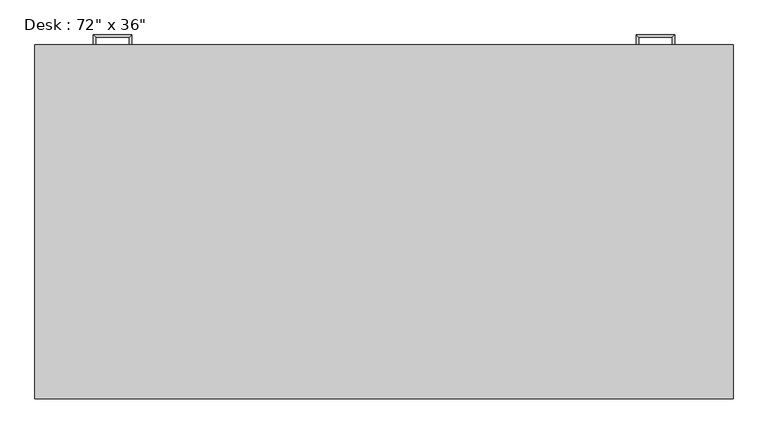
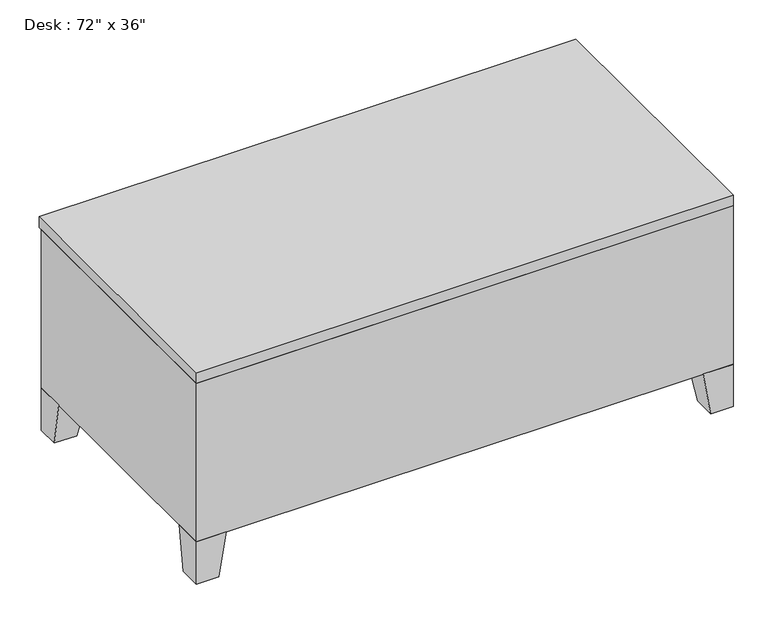
"""IFC4 building model written with IfcOpenShell, lengths in millimetres: furniture geometry."""

from ifc_helpers import new_model, si_unit, frame, origin, place, context, project, spatial, polyline, outline, extrude, faceted_brep, source, transform, mapped, element, save


def furniture_65204735(model_context):
    return source(origin(), model_context, "Body", "SolidModel", [
        extrude(outline(polyline([(-133.35, 76.2), (-133.35, 88.9), (234.95, 88.9), (234.95, 76.2), (-133.35, 76.2)])), frame((0.0, 0.0, 603.25), z_axis=(0.0, 0.0, 1.0), x_axis=(1.0, 0.0, 0.0)), (0.0, 0.0, 1.0), 101.6),
        extrude(outline(polyline([(-133.35, 76.2), (-133.35, 88.9), (234.95, 88.9), (234.95, 76.2), (-133.35, 76.2)])), frame((0.0, 0.0, 171.45), z_axis=(0.0, 0.0, 1.0), x_axis=(1.0, 0.0, 0.0)), (0.0, 0.0, 1.0), 412.75),
        extrude(outline(polyline([(1289.05, 76.2), (1289.05, 88.9), (1657.35, 88.9), (1657.35, 76.2), (1289.05, 76.2)])), frame((0.0, 0.0, 603.25), z_axis=(0.0, 0.0, 1.0), x_axis=(1.0, 0.0, 0.0)), (0.0, 0.0, 1.0), 101.6),
        extrude(outline(polyline([(1289.05, 76.2), (1289.05, 88.9), (1657.35, 88.9), (1657.35, 76.2), (1289.05, 76.2)])), frame((0.0, 0.0, 171.45), z_axis=(0.0, 0.0, 1.0), x_axis=(1.0, 0.0, 0.0)), (0.0, 0.0, 1.0), 171.45),
        extrude(outline(polyline([(1289.05, 76.2), (1289.05, 88.9), (1657.35, 88.9), (1657.35, 76.2), (1289.05, 76.2)])), frame((0.0, 0.0, 482.6), z_axis=(0.0, 0.0, 1.0), x_axis=(1.0, 0.0, 0.0)), (0.0, 0.0, 1.0), 101.6),
        extrude(outline(polyline([(1289.05, 76.2), (1289.05, 88.9), (1657.35, 88.9), (1657.35, 76.2), (1289.05, 76.2)])), frame((0.0, 0.0, 361.95), z_axis=(0.0, 0.0, 1.0), x_axis=(1.0, 0.0, 0.0)), (0.0, 0.0, 1.0), 101.6),
        faceted_brep([(-50.8, 76.2, 152.4), (-152.4, 76.2, 152.4), (-152.4, -25.4, 152.4), (-50.8, -25.4, 152.4), (-76.2, 76.2, 0.0), (-76.2, 0.0, 0.0), (-152.4, 0.0, 0.0), (-152.4, 76.2, 0.0)], [[[0, 1, 2, 3]], [[4, 5, 6, 7]], [[4, 0, 3, 5]], [[5, 3, 2, 6]], [[6, 2, 1, 7]], [[7, 1, 0, 4]]]),
        faceted_brep([(-50.8, -838.2, 152.4), (-50.8, -736.6, 152.4), (-152.4, -736.6, 152.4), (-152.4, -838.2, 152.4), (-76.2, -838.2, 0.0), (-152.4, -838.2, 0.0), (-152.4, -762.0, 0.0), (-76.2, -762.0, 0.0)], [[[0, 1, 2, 3]], [[4, 5, 6, 7]], [[4, 0, 3, 5]], [[5, 3, 2, 6]], [[6, 2, 1, 7]], [[7, 1, 0, 4]]]),
        faceted_brep([(1574.8, -838.2, 152.4), (1676.4, -838.2, 152.4), (1676.4, -736.6, 152.4), (1574.8, -736.6, 152.4), (1600.2, -838.2, 0.0), (1600.2, -762.0, 0.0), (1676.4, -762.0, 0.0), (1676.4, -838.2, 0.0)], [[[0, 1, 2, 3]], [[4, 5, 6, 7]], [[4, 0, 3, 5]], [[5, 3, 2, 6]], [[6, 2, 1, 7]], [[7, 1, 0, 4]]]),
        faceted_brep([(1574.8, 76.2, 152.4), (1574.8, -25.4, 152.4), (1676.4, -25.4, 152.4), (1676.4, 76.2, 152.4), (1600.2, 76.2, 0.0), (1676.4, 76.2, 0.0), (1676.4, 0.0, 0.0), (1600.2, 0.0, 0.0)], [[[0, 1, 2, 3]], [[4, 5, 6, 7]], [[4, 0, 3, 5]], [[5, 3, 2, 6]], [[6, 2, 1, 7]], [[7, 1, 0, 4]]]),
        extrude(outline(polyline([(-152.4, 88.9), (1676.4, 88.9), (1676.4, -838.2), (-152.4, -838.2), (-152.4, 88.9)])), frame((0.0, 0.0, 723.9), z_axis=(0.0, 0.0, 1.0), x_axis=(1.0, 0.0, 0.0)), (0.0, 0.0, 1.0), 38.1),
        extrude(outline(polyline([(1270.0, 76.2), (1676.4, 76.2), (1676.4, -838.2), (-152.4, -838.2), (-152.4, 76.2), (254.0, 76.2), (254.0, -711.2), (1270.0, -711.2), (1270.0, 76.2)])), frame((0.0, 0.0, 152.4), z_axis=(0.0, 0.0, 1.0), x_axis=(1.0, 0.0, 0.0)), (0.0, 0.0, 1.0), 571.5),
        faceted_brep([(6.35, 88.9, 546.1), (0.0, 88.9, 546.1), (0.0, 88.9, 533.4), (6.35, 88.9, 533.4), (6.35, 107.95, 533.4), (6.35, 107.95, 546.1), (0.0, 114.3, 533.4), (0.0, 114.3, 546.1), (95.25, 107.95, 533.4), (95.25, 107.95, 546.1), (101.6, 114.3, 533.4), (101.6, 114.3, 546.1), (95.25, 88.9, 546.1), (95.25, 88.9, 533.4), (101.6, 88.9, 533.4), (101.6, 88.9, 546.1)], [[[0, 1, 2, 3]], [[3, 4, 5, 0]], [[2, 6, 4, 3]], [[1, 7, 6, 2]], [[0, 5, 7, 1]], [[4, 8, 9, 5]], [[6, 10, 8, 4]], [[7, 11, 10, 6]], [[5, 9, 11, 7]], [[12, 13, 14, 15]], [[8, 13, 12, 9]], [[10, 14, 13, 8]], [[11, 15, 14, 10]], [[9, 12, 15, 11]]]),
        faceted_brep([(6.35, 88.9, 666.75), (0.0, 88.9, 666.75), (0.0, 88.9, 654.05), (6.35, 88.9, 654.05), (6.35, 107.95, 654.05), (6.35, 107.95, 666.75), (0.0, 114.3, 654.05), (0.0, 114.3, 666.75), (95.25, 107.95, 654.05), (95.25, 107.95, 666.75), (101.6, 114.3, 654.05), (101.6, 114.3, 666.75), (95.25, 88.9, 666.75), (95.25, 88.9, 654.05), (101.6, 88.9, 654.05), (101.6, 88.9, 666.75)], [[[0, 1, 2, 3]], [[3, 4, 5, 0]], [[2, 6, 4, 3]], [[1, 7, 6, 2]], [[0, 5, 7, 1]], [[4, 8, 9, 5]], [[6, 10, 8, 4]], [[7, 11, 10, 6]], [[5, 9, 11, 7]], [[12, 13, 14, 15]], [[8, 13, 12, 9]], [[10, 14, 13, 8]], [[11, 15, 14, 10]], [[9, 12, 15, 11]]]),
        faceted_brep([(1517.65, 88.9, 304.8), (1517.65, 88.9, 292.1), (1524.0, 88.9, 292.1), (1524.0, 88.9, 304.8), (1524.0, 114.3, 304.8), (1517.65, 107.95, 304.8), (1524.0, 114.3, 292.1), (1517.65, 107.95, 292.1), (1422.4, 114.3, 304.8), (1428.75, 107.95, 304.8), (1422.4, 114.3, 292.1), (1428.75, 107.95, 292.1), (1428.75, 88.9, 304.8), (1422.4, 88.9, 304.8), (1422.4, 88.9, 292.1), (1428.75, 88.9, 292.1)], [[[0, 1, 2, 3]], [[3, 4, 5, 0]], [[2, 6, 4, 3]], [[1, 7, 6, 2]], [[0, 5, 7, 1]], [[4, 8, 9, 5]], [[6, 10, 8, 4]], [[7, 11, 10, 6]], [[5, 9, 11, 7]], [[12, 13, 14, 15]], [[8, 13, 12, 9]], [[10, 14, 13, 8]], [[11, 15, 14, 10]], [[9, 12, 15, 11]]]),
        faceted_brep([(1517.65, 88.9, 425.45), (1517.65, 88.9, 412.75), (1524.0, 88.9, 412.75), (1524.0, 88.9, 425.45), (1524.0, 114.3, 425.45), (1517.65, 107.95, 425.45), (1524.0, 114.3, 412.75), (1517.65, 107.95, 412.75), (1422.4, 114.3, 425.45), (1428.75, 107.95, 425.45), (1422.4, 114.3, 412.75), (1428.75, 107.95, 412.75), (1428.75, 88.9, 425.45), (1422.4, 88.9, 425.45), (1422.4, 88.9, 412.75), (1428.75, 88.9, 412.75)], [[[0, 1, 2, 3]], [[3, 4, 5, 0]], [[2, 6, 4, 3]], [[1, 7, 6, 2]], [[0, 5, 7, 1]], [[4, 8, 9, 5]], [[6, 10, 8, 4]], [[7, 11, 10, 6]], [[5, 9, 11, 7]], [[12, 13, 14, 15]], [[8, 13, 12, 9]], [[10, 14, 13, 8]], [[11, 15, 14, 10]], [[9, 12, 15, 11]]]),
        faceted_brep([(1517.65, 88.9, 546.1), (1517.65, 88.9, 533.4), (1524.0, 88.9, 533.4), (1524.0, 88.9, 546.1), (1524.0, 114.3, 546.1), (1517.65, 107.95, 546.1), (1524.0, 114.3, 533.4), (1517.65, 107.95, 533.4), (1422.4, 114.3, 546.1), (1428.75, 107.95, 546.1), (1422.4, 114.3, 533.4), (1428.75, 107.95, 533.4), (1428.75, 88.9, 546.1), (1422.4, 88.9, 546.1), (1422.4, 88.9, 533.4), (1428.75, 88.9, 533.4)], [[[0, 1, 2, 3]], [[3, 4, 5, 0]], [[2, 6, 4, 3]], [[1, 7, 6, 2]], [[0, 5, 7, 1]], [[4, 8, 9, 5]], [[6, 10, 8, 4]], [[7, 11, 10, 6]], [[5, 9, 11, 7]], [[12, 13, 14, 15]], [[8, 13, 12, 9]], [[10, 14, 13, 8]], [[11, 15, 14, 10]], [[9, 12, 15, 11]]]),
        faceted_brep([(1517.65, 88.9, 666.75), (1517.65, 88.9, 654.05), (1524.0, 88.9, 654.05), (1524.0, 88.9, 666.75), (1524.0, 114.3, 666.75), (1517.65, 107.95, 666.75), (1524.0, 114.3, 654.05), (1517.65, 107.95, 654.05), (1422.4, 114.3, 666.75), (1428.75, 107.95, 666.75), (1422.4, 114.3, 654.05), (1428.75, 107.95, 654.05), (1428.75, 88.9, 666.75), (1422.4, 88.9, 666.75), (1422.4, 88.9, 654.05), (1428.75, 88.9, 654.05)], [[[0, 1, 2, 3]], [[3, 4, 5, 0]], [[2, 6, 4, 3]], [[1, 7, 6, 2]], [[0, 5, 7, 1]], [[4, 8, 9, 5]], [[6, 10, 8, 4]], [[7, 11, 10, 6]], [[5, 9, 11, 7]], [[12, 13, 14, 15]], [[8, 13, 12, 9]], [[10, 14, 13, 8]], [[11, 15, 14, 10]], [[9, 12, 15, 11]]]),
    ])


if __name__ == "__main__":
    model = new_model("IFC4")
    model_context = context("Model", 3, world=origin())
    ifc_project = project(units=[si_unit("LENGTHUNIT", "METRE", prefix="MILLI")], contexts=[model_context])
    site = spatial("IfcSite", under=ifc_project)
    building = spatial("IfcBuilding", under=site)
    placement = place(None, origin())
    furniture_shape = furniture_65204735(model_context)
    element("IfcFurniture", 1, ObjectType="Desk : 72\" x 36\"", at=placement, inside=building, context=model_context, shape_type="MappedRepresentation", body=[
        mapped(furniture_shape, transform((0.0, 0.0, 0.0), x_axis=(1.0, 0.0, 0.0), y_axis=(0.0, 1.0, 0.0), z_axis=(0.0, 0.0, 1.0))),
    ])
    save(model, "model.ifc")

# Revit data of these elements
# Type "Desk : 72\" x 36\""
#   Assembly Code = "E2020200"
#   Depth = 3' - 0"
#   Height = 2' - 6"
#   Leg Height = 0' - 6"
#   Width = 6' - 0"
#   Body Material = Laminate, Ivory, Matte
#   Handle/Leg Material = Steel, Chrome Plated
#   Top Material = Cherry
#   Default Elevation = 0
# Element 1 (IfcFurniture, "Desk : 72\" x 36\"")
#   Materials on its faces: "Steel, Chrome Plated", "Laminate, Ivory, Matte", "Cherry"
# Materials
#   "Laminate, Ivory, Matte": class "Plastic", colour RGB 247 247 239, transparency 0, Description = "Plastic Laminate - Ivory, Matte", Cost = 0
#   "Steel, Chrome Plated": class "Metal", colour RGB 17 17 17, transparency 0, Description = "Chromiuim plated steel", Cost = 0
#   "Cherry": class "Wood", colour RGB 226 177 128, transparency 0, Description = "Prunus Serotina", Cost = 0
